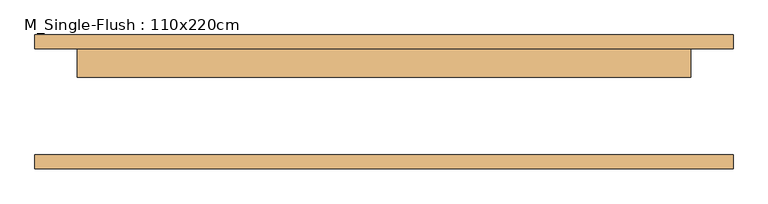
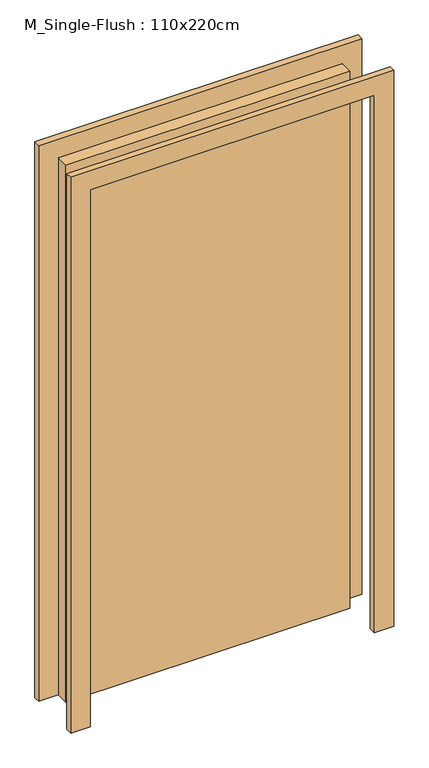
"""IFC4 building model written with IfcOpenShell, lengths in millimetres: door geometry, M_Single-Flush : 110x220cm."""

from ifc_helpers import new_model, si_unit, frame, origin, origin_with_axes, place, context, project, spatial, polyline, outline, extrude, source, transform, mapped, element, save


def m_single_flush_110x220cm_1748ef91(model_context):
    return source(origin(), model_context, "Body", "SweptSolid", [
        extrude(outline(polyline([(2276.0, -626.0), (0.0, -626.0), (0.0, -550.0), (2200.0, -550.0), (2200.0, 550.0), (0.0, 550.0), (0.0, 626.0), (2276.0, 626.0), (2276.0, -626.0)])), frame((0.0, 95.0, 0.0), z_axis=(0.0, 1.0, 0.0), x_axis=(0.0, 0.0, 1.0)), (0.0, 0.0, 1.0), 25.0),
        extrude(outline(polyline([(2276.0, 626.0), (2276.0, -626.0), (0.0, -626.0), (0.0, -550.0), (2200.0, -550.0), (2200.0, 550.0), (0.0, 550.0), (0.0, 626.0), (2276.0, 626.0)])), frame((0.0, -120.0, 0.0), z_axis=(0.0, 1.0, 0.0), x_axis=(0.0, 0.0, 1.0)), (0.0, 0.0, 1.0), 25.0),
        extrude(outline(polyline([(550.0, 44.0), (-550.0, 44.0), (-550.0, 95.0), (550.0, 95.0), (550.0, 44.0)])), origin_with_axes(), (0.0, 0.0, 1.0), 2200.0),
    ])


if __name__ == "__main__":
    model = new_model("IFC4")
    model_context = context("Model", 3, world=origin())
    ifc_project = project(units=[si_unit("LENGTHUNIT", "METRE", prefix="MILLI")], contexts=[model_context])
    site = spatial("IfcSite", under=ifc_project)
    building = spatial("IfcBuilding", under=site)
    placement = place(None, origin())
    m_single_flush_110x220cm_shape = m_single_flush_110x220cm_1748ef91(model_context)
    element("IfcDoor", 1, ObjectType="M_Single-Flush : 110x220cm", at=placement, inside=building, context=model_context, shape_type="MappedRepresentation", body=[
        mapped(m_single_flush_110x220cm_shape, transform((0.0, 0.0, 0.0), x_axis=(1.0, 0.0, 0.0), y_axis=(0.0, 1.0, 0.0), z_axis=(0.0, 0.0, 1.0))),
    ])
    save(model, "model.ifc")

# Revit data of these elements
# Type "M_Single-Flush : 110x220cm"
#   Type Mark = "45"
#   Construction Type Id = "MDOOR"
#   Analytic Construction = "Metal"
#   Thickness = 5.10 cm
#   Heat Transfer Coefficient (U) = 3.7021 W/(m²·K)
#   Height = 220.00 cm
#   Trim Projection Ext = 2.50 cm
#   Trim Projection Int = 2.50 cm
#   Trim Width = 7.60 cm
#   Width = 110.00 cm
#   Define Thermal Properties by = 1
#   Door Material = Door - Panel
#   Frame Material = Door - Frame
#   Visual Light Transmittance = 0
#   Solar Heat Gain Coefficient = 0
#   Function = (empty or 0)
#   Wall Closure = (empty or 0)
# Element 1 (IfcDoor, "M_Single-Flush : 110x220cm")
#   Materials on its faces: "Door - Frame", "Door - Panel"
# Materials
#   "Door - Panel": class "Wood", colour RGB 210 159 95, transparency 0, Cost = 0
#   "Door - Frame": class "Miscellaneous", colour RGB 118 70 51, transparency 0, Cost = 0
